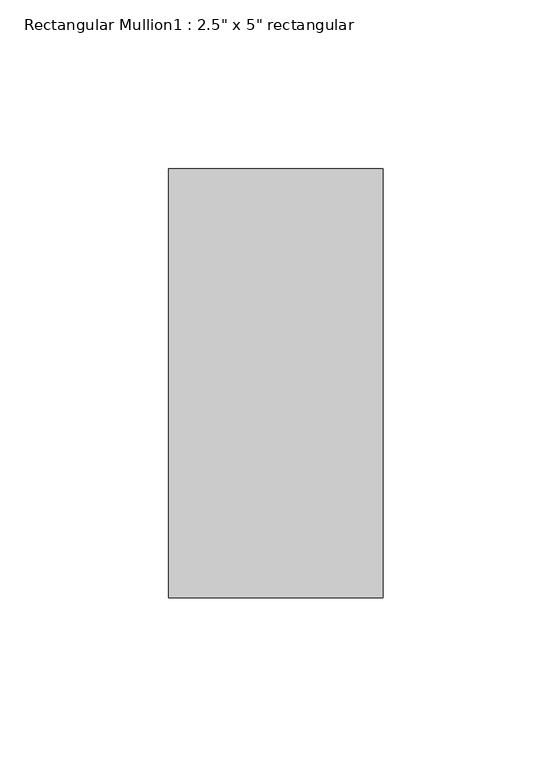
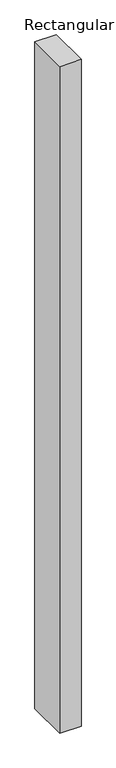
"""IFC4 building model written with IfcOpenShell, lengths in millimetres: member geometry."""

from ifc_helpers import new_model, si_unit, frame, origin, place, context, project, spatial, polyline, outline, extrude, source, transform, mapped, element, save


def member_a397286f(model_context):
    return source(origin(), model_context, "Body", "SweptSolid", [
        extrude(outline(polyline([(0.0, 63.5), (0.0, -63.5), (-63.5, -63.5), (-63.5, 63.5), (0.0, 63.5)])), frame((0.0, 0.0, -2091.69), z_axis=(0.0, 0.0, 1.0), x_axis=(1.0, 0.0, 0.0)), (0.0, 0.0, 1.0), 2091.69),
    ])


if __name__ == "__main__":
    model = new_model("IFC4")
    model_context = context("Model", 3, world=origin())
    ifc_project = project(units=[si_unit("LENGTHUNIT", "METRE", prefix="MILLI")], contexts=[model_context])
    site = spatial("IfcSite", under=ifc_project)
    building = spatial("IfcBuilding", under=site)
    placement = place(None, origin())
    member_shape = member_a397286f(model_context)
    element("IfcMember", 1, ObjectType="Rectangular Mullion1 : 2.5\" x 5\" rectangular", at=placement, inside=building, context=model_context, shape_type="MappedRepresentation", body=[
        mapped(member_shape, transform((0.0, 0.0, 0.0), x_axis=(1.0, 0.0, 0.0), y_axis=(0.0, 1.0, 0.0), z_axis=(0.0, 0.0, 1.0))),
    ])
    save(model, "model.ifc")

# Revit data of these elements
# Type "Rectangular Mullion1 : 2.5\" x 5\" rectangular"
#   built-in parameter 1007304 = 0.416667 (stored number, unit not read)
#   built-in parameter 1007301 = 0.104167 (stored number, unit not read)
#   built-in parameter 1007300 = 0.104167 (stored number, unit not read)
# Element 1 (IfcMember, "Rectangular Mullion1 : 2.5\" x 5\" rectangular")
#   Materials on its faces: "support-frame"
# Materials
#   "support-frame": class "Unassigned", colour RGB 233 233 233, transparency 0, Cost = 0
